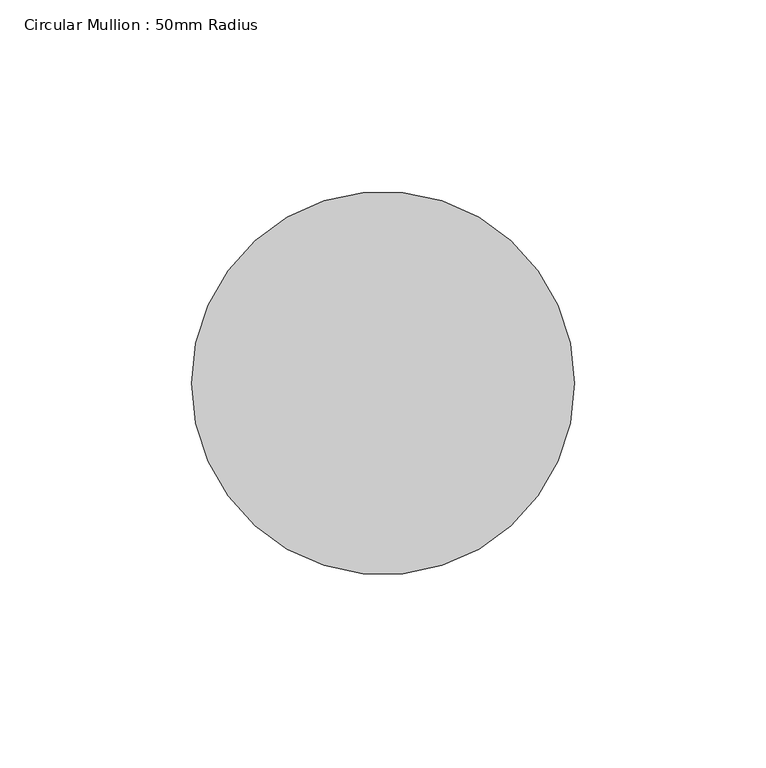
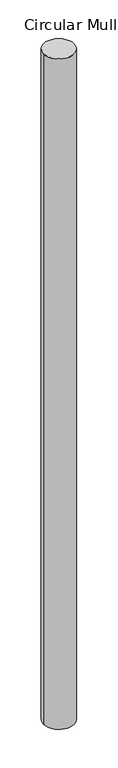
"""IFC4 building model written with IfcOpenShell, lengths in millimetres: member geometry, Circular Mullion : 50mm Radius."""

from ifc_helpers import new_model, si_unit, point, frame, origin, origin_2d, place, context, project, spatial, circle_curve, trimmed, segment, composite_curve, outline, extrude, source, transform, mapped, element, save


def circular_mullion_50mm_radius_3d6b8998(model_context):
    return source(origin(), model_context, "Body", "SweptSolid", [
        extrude(outline(composite_curve([segment(trimmed(circle_curve(origin_2d(), 50.0), [point((50.0, 0.0))], [point((-50.0, 0.0))], False, "CARTESIAN"), True, "CONTINUOUS"), segment(trimmed(circle_curve(origin_2d(), 50.0), [point((-50.0, 0.0))], [point((50.0, 0.0))], False, "CARTESIAN"), True, "CONTINUOUS")], self_intersect=False)), frame((0.0, 0.0, -2310.2958618), z_axis=(0.0, 0.0, 1.0), x_axis=(1.0, 0.0, 0.0)), (0.0, 0.0, 1.0), 2310.2958618),
    ])


if __name__ == "__main__":
    model = new_model("IFC4")
    model_context = context("Model", 3, world=origin())
    ifc_project = project(units=[si_unit("LENGTHUNIT", "METRE", prefix="MILLI")], contexts=[model_context])
    site = spatial("IfcSite", under=ifc_project)
    building = spatial("IfcBuilding", under=site)
    placement = place(None, origin())
    circular_mullion_50mm_radius_shape = circular_mullion_50mm_radius_3d6b8998(model_context)
    element("IfcMember", 1, ObjectType="Circular Mullion : 50mm Radius", at=placement, inside=building, context=model_context, shape_type="MappedRepresentation", body=[
        mapped(circular_mullion_50mm_radius_shape, transform((0.0, 0.0, 0.0), x_axis=(1.0, 0.0, 0.0), y_axis=(0.0, 1.0, 0.0), z_axis=(0.0, 0.0, 1.0))),
    ])
    save(model, "model.ifc")

# Revit data of these elements
# Type "Circular Mullion : 50mm Radius"
#   built-in parameter 1007350 = 0.164042 (stored number, unit not read)
# Element 1 (IfcMember, "Circular Mullion : 50mm Radius")
#   Materials on its faces: "Aluminium"
# Materials
#   "Aluminium": class "Metal", colour RGB 247 247 247, transparency 0, Description = "Aluminium 6061", Cost = 0
